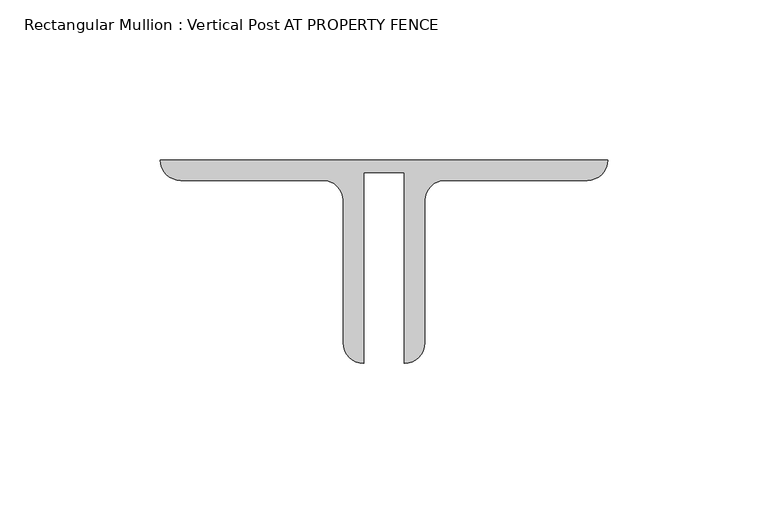
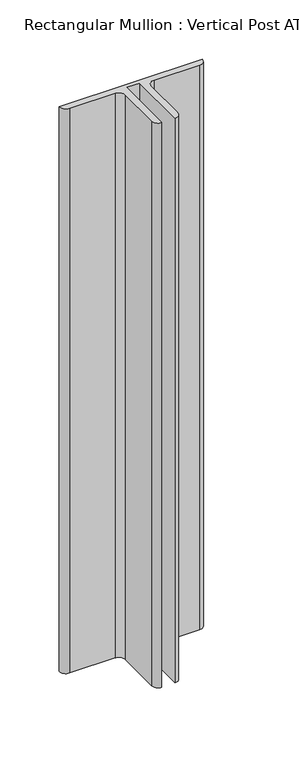
"""IFC4 building model written with IfcOpenShell, lengths in millimetres: member geometry, Rectangular Mullion : Vertical Post AT PROPERTY FENCE."""

from ifc_helpers import new_model, si_unit, point, frame, frame_2d, origin, place, context, project, spatial, polyline, circle_curve, trimmed, segment, composite_curve, outline, extrude, source, transform, mapped, element, save


def rectangular_mullion_vertical_post_at_property_fence_8fdf4037(model_context):
    return source(origin(), model_context, "Body", "SweptSolid", [
        extrude(outline(composite_curve([segment(polyline([(-76.2, -22.9145205), (-76.2, -82.55)]), True, "CONTINUOUS"), segment(trimmed(circle_curve(frame_2d((-76.2, -76.2)), 6.35), [point((-76.2, -82.55))], [point((-82.55, -76.2))], False, "CARTESIAN"), True, "CONTINUOUS"), segment(polyline([(-82.55, -76.2), (-82.55, -31.75)]), True, "CONTINUOUS"), segment(trimmed(circle_curve(frame_2d((-88.9, -31.75)), 6.35), [point((-82.55, -31.75))], [point((-88.9, -25.4))], True, "CARTESIAN"), True, "CONTINUOUS"), segment(polyline([(-88.9, -25.4), (-133.35, -25.4)]), True, "CONTINUOUS"), segment(trimmed(circle_curve(frame_2d((-133.35, -19.05)), 6.35), [point((-133.35, -25.4))], [point((-139.7, -19.05))], False, "CARTESIAN"), True, "CONTINUOUS"), segment(polyline([(-139.7, -19.05), (0.0, -19.05)]), True, "CONTINUOUS"), segment(trimmed(circle_curve(frame_2d((-6.35, -19.05)), 6.35), [point((0.0, -19.05))], [point((-6.35, -25.4))], False, "CARTESIAN"), True, "CONTINUOUS"), segment(polyline([(-6.35, -25.4), (-50.8, -25.4)]), True, "CONTINUOUS"), segment(trimmed(circle_curve(frame_2d((-50.8, -31.75)), 6.35), [point((-50.8, -25.4))], [point((-57.15, -31.75))], True, "CARTESIAN"), True, "CONTINUOUS"), segment(polyline([(-57.15, -31.75), (-57.15, -76.2)]), True, "CONTINUOUS"), segment(trimmed(circle_curve(frame_2d((-63.5, -76.2)), 6.35), [point((-57.15, -76.2))], [point((-63.5, -82.55))], False, "CARTESIAN"), True, "CONTINUOUS"), segment(polyline([(-63.5, -82.55), (-63.5, -22.9145205), (-76.2, -22.9145205)]), True, "CONTINUOUS")], self_intersect=False)), frame((0.0, 0.0, -581.9336948), z_axis=(0.0, 0.0, 1.0), x_axis=(1.0, 0.0, 0.0)), (0.0, 0.0, 1.0), 581.9336948),
    ])


if __name__ == "__main__":
    model = new_model("IFC4")
    model_context = context("Model", 3, world=origin())
    ifc_project = project(units=[si_unit("LENGTHUNIT", "METRE", prefix="MILLI")], contexts=[model_context])
    site = spatial("IfcSite", under=ifc_project)
    building = spatial("IfcBuilding", under=site)
    placement = place(None, origin())
    rectangular_mullion_vertical_post_at_property_fence_shape = rectangular_mullion_vertical_post_at_property_fence_8fdf4037(model_context)
    element("IfcMember", 1, ObjectType="Rectangular Mullion : Vertical Post AT PROPERTY FENCE", at=placement, inside=building, context=model_context, shape_type="MappedRepresentation", body=[
        mapped(rectangular_mullion_vertical_post_at_property_fence_shape, transform((0.0, 0.0, 0.0), x_axis=(1.0, 0.0, 0.0), y_axis=(0.0, 1.0, 0.0), z_axis=(0.0, 0.0, 1.0))),
    ])
    save(model, "model.ifc")

# Revit data of these elements
# Type "Rectangular Mullion : Vertical Post AT PROPERTY FENCE"
#   built-in parameter 1007351 = -0.0625 (stored number, unit not read)
#   built-in parameter 1007322 = 0.0126789 (stored number, unit not read)
#   built-in parameter 1007321 = 0.229167 (stored number, unit not read)
#   built-in parameter 1007320 = 0.229167 (stored number, unit not read)
# Element 1 (IfcMember, "Rectangular Mullion : Vertical Post AT PROPERTY FENCE")
#   Materials on its faces: "MAIN FENCE POST: (2) BACK/BACK GALVANIZED ANGLES (2) L2 1/2 X 2 1/2 X 1/4\") ANCHORED TO 8\"W X 42\" DEEP CONCRETE FOOTING(1)"
# Materials
#   "MAIN FENCE POST: (2) BACK/BACK GALVANIZED ANGLES (2) L2 1/2 X 2 1/2 X 1/4\") ANCHORED TO 8\"W X 42\" DEEP CONCRETE FOOTING(1)": class "Unassigned", colour RGB 211 211 211, transparency 0, Cost = 0
